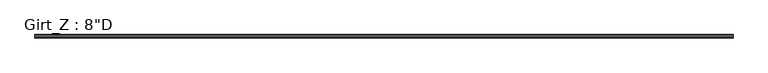
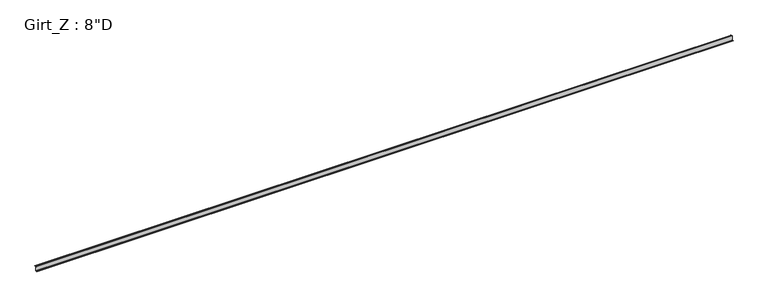
"""IFC4 building model written with IfcOpenShell, lengths in millimetres: beam geometry."""

from ifc_helpers import new_model, si_unit, point, frame, frame_2d, origin, place, context, project, spatial, polyline, circle_curve, trimmed, segment, composite_curve, outline, extrude, source, transform, mapped, element, save


def beam_fadfea3b(model_context):
    return source(origin(), model_context, "Body", "SweptSolid", [
        extrude(outline(composite_curve([segment(polyline([(63.5, 101.6), (75.745104, 87.0068534), (73.6169367, 85.221109), (62.204539, 98.821875), (3.3005807, 98.821875)]), True, "CONTINUOUS"), segment(trimmed(circle_curve(frame_2d((3.3741066, 96.8381931)), 1.9850441), [point((3.3005807, 98.821875))], [point((1.3890625, 96.8381931))], True, "CARTESIAN"), True, "CONTINUOUS"), segment(polyline([(1.3890625, 96.8381931), (1.3890625, -96.8375)]), True, "CONTINUOUS"), segment(trimmed(circle_curve(frame_2d((-3.3734375, -96.8375)), 4.7625), [point((1.3890625, -96.8375))], [point((-3.3734375, -101.6))], False, "CARTESIAN"), True, "CONTINUOUS"), segment(polyline([(-3.3734375, -101.6), (-63.5, -101.6), (-75.745104, -87.0068534), (-73.6169367, -85.221109), (-62.204539, -98.821875), (-3.2694106, -98.821875)]), True, "CONTINUOUS"), segment(trimmed(circle_curve(frame_2d((-3.3748024, -96.8389339)), 1.9857399), [point((-3.2694106, -98.821875))], [point((-1.3890625, -96.8389339))], True, "CARTESIAN"), True, "CONTINUOUS"), segment(polyline([(-1.3890625, -96.8389339), (-1.3890625, 96.8375)]), True, "CONTINUOUS"), segment(trimmed(circle_curve(frame_2d((3.3734375, 96.8375)), 4.7625), [point((-1.3890625, 96.8375))], [point((3.3734375, 101.6))], False, "CARTESIAN"), True, "CONTINUOUS"), segment(polyline([(3.3734375, 101.6), (63.5, 101.6)]), True, "CONTINUOUS")], self_intersect=False)), frame((-15595.6, 0.0, 0.0), z_axis=(1.0, 0.0, 0.0), x_axis=(0.0, 1.0, 0.0)), (0.0, 0.0, 1.0), 31191.2),
    ])


if __name__ == "__main__":
    model = new_model("IFC4")
    model_context = context("Model", 3, world=origin())
    ifc_project = project(units=[si_unit("LENGTHUNIT", "METRE", prefix="MILLI")], contexts=[model_context])
    site = spatial("IfcSite", under=ifc_project)
    building = spatial("IfcBuilding", under=site)
    placement = place(None, origin())
    beam_shape = beam_fadfea3b(model_context)
    element("IfcBeam", 1, ObjectType="Girt_Z : 8\"D", at=placement, inside=building, context=model_context, shape_type="MappedRepresentation", body=[
        mapped(beam_shape, transform((0.0, 0.0, 0.0), x_axis=(1.0, 0.0, 0.0), y_axis=(0.0, 1.0, 0.0), z_axis=(0.0, 0.0, 1.0))),
    ])
    save(model, "model.ifc")

# Revit data of these elements
# Type "Girt_Z : 8\"D"
#   Web_Thickness = 0' - 0 7/64"
#   Length [instance default] = 10' - 0"
#   Leg_1 = 0' - 2 1/2"
#   Height = 0' - 8"
#   Structural Material [instance default] = none
# Element 1 (IfcBeam, "Girt_Z : 8\"D")
#   Structural Material = Steel
#   Materials on its faces: "Steel"
# Materials
#   "Steel": class "Metal", colour RGB 118 118 114, transparency 0, Description = "Steel, mill finish", Cost = 0
